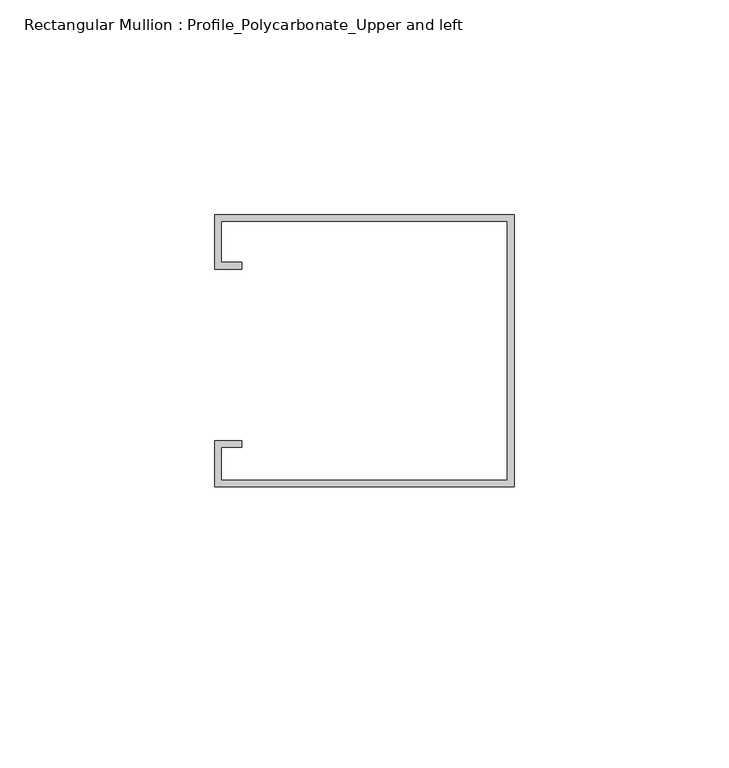
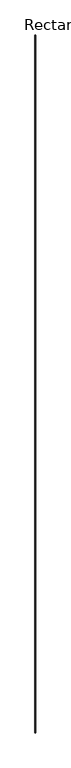
"""IFC4 building model written with IfcOpenShell, lengths in millimetres: member geometry, Rectangular Mullion : Profile_Polycarbonate_Upper and left."""

import ifcopenshell
import ifcopenshell.guid

model = None  # the IFC model being written
_history = None  # IfcOwnerHistory: only IFC2X3 demands one
_inside = {}  # id of a spatial element -> (the spatial element, [elements in it])
_under = {}  # id of a project, library or spatial element -> (it, [spatial elements below it])
_declared = {}  # id of a project -> (the project, [libraries it declares])
_typed = {}  # id of a type object -> (the type object, [elements of that type])
_made_of = {}  # id of a material, layer set ... -> (it, [elements and type objects made of it])


def new_model(schema):
    """Start an empty IFC model of exactly this schema.

    Asked for "IFC4X3", IfcOpenShell would pick the latest addendum, in which some entities
    have other attributes; the version numbers below select the first issue.
    IFC2X3 requires an IfcOwnerHistory on every rooted entity: one is made here for all.
    """
    global model, _history
    if schema == "IFC4X3":
        model = ifcopenshell.file(schema_version=(4, 3, 0, 0))
    else:
        model = ifcopenshell.file(schema=schema)
    _inside.clear()
    _under.clear()
    _declared.clear()
    _typed.clear()
    _made_of.clear()
    _history = None
    if model.schema == "IFC2X3":
        org = make("IfcOrganization", Name="unknown")
        user = make(
            "IfcPersonAndOrganization",
            ThePerson=make("IfcPerson", FamilyName="unknown"),
            TheOrganization=org,
        )
        app = make(
            "IfcApplication",
            ApplicationDeveloper=org,
            Version="unknown",
            ApplicationFullName="unknown",
            ApplicationIdentifier="unknown",
        )
        _history = make(
            "IfcOwnerHistory",
            OwningUser=user,
            OwningApplication=app,
            ChangeAction="ADDED",
            CreationDate=0,
        )
    return model


def make(cls, **values):
    """One entity of the class cls with the attributes given. An attribute that is None is left unset."""
    return model.create_entity(
        cls, **{name: value for name, value in values.items() if value is not None}
    )


def rooted(cls, **values):
    """An entity with a GlobalId (a new one), such as an element, a storey or a relation."""
    return make(cls, GlobalId=ifcopenshell.guid.new(), OwnerHistory=_history, **values)


def si_unit(unit_type, name, prefix=None):
    """IfcSIUnit, for example si_unit("LENGTHUNIT", "METRE", prefix="MILLI")."""
    return make("IfcSIUnit", UnitType=unit_type, Prefix=prefix, Name=name)


def assignment(units):
    """IfcUnitAssignment: the units of a project."""
    return None if units is None else make("IfcUnitAssignment", Units=units)


def point(xyz):
    """IfcCartesianPoint."""
    return None if xyz is None else make("IfcCartesianPoint", Coordinates=xyz)


def direction(xyz):
    """IfcDirection."""
    return None if xyz is None else make("IfcDirection", DirectionRatios=xyz)


def frame(location, z_axis=None, x_axis=None):
    """IfcAxis2Placement3D, a coordinate frame: its origin and axes. An axis left out is left unset."""
    return make(
        "IfcAxis2Placement3D",
        Location=point(location),
        Axis=direction(z_axis),
        RefDirection=direction(x_axis),
    )


def origin():
    """The frame at (0, 0, 0) with its axes left unset."""
    return frame((0.0, 0.0, 0.0))


def place(relative_to, where):
    """IfcLocalPlacement: puts the frame where relative to a parent placement (None: the world)."""
    return make(
        "IfcLocalPlacement", PlacementRelTo=relative_to, RelativePlacement=where
    )


def context(
    kind, dimensions, precision=None, world=None, true_north=None, identifier=None
):
    """IfcGeometricRepresentationContext, for example the 3D "Model" context."""
    return make(
        "IfcGeometricRepresentationContext",
        ContextIdentifier=identifier,
        ContextType=kind,
        CoordinateSpaceDimension=dimensions,
        Precision=precision,
        WorldCoordinateSystem=world,
        TrueNorth=true_north,
    )


def project(units=None, contexts=None):
    """IfcProject with its units and contexts."""
    return rooted(
        "IfcProject",
        Name="project",
        RepresentationContexts=contexts,
        UnitsInContext=assignment(units),
    )


def spatial(cls, under=None, at=None, **own):
    """A site, building, storey or space (cls), placed at a placement, below another one or the project."""
    s = rooted(cls, ObjectPlacement=at, **own)
    if under is not None:
        _under.setdefault(under.id(), (under, []))[1].append(s)
    return s


def polyline(points):
    """IfcPolyline through the points."""
    return make("IfcPolyline", Points=[point(p) for p in points])


def outline(outer, holes=None, kind="AREA"):
    """IfcArbitraryClosedProfileDef: a profile drawn as a closed curve; with holes, ...WithVoids."""
    if holes is None:
        return make("IfcArbitraryClosedProfileDef", ProfileType=kind, OuterCurve=outer)
    return make(
        "IfcArbitraryProfileDefWithVoids",
        ProfileType=kind,
        OuterCurve=outer,
        InnerCurves=holes,
    )


def extrude(swept, where, along, depth):
    """IfcExtrudedAreaSolid: the profile swept, set in the frame where, extruded along a direction by depth."""
    return make(
        "IfcExtrudedAreaSolid",
        SweptArea=swept,
        Position=where,
        ExtrudedDirection=direction(along),
        Depth=depth,
    )


def shape(context_of_items, identifier, shape_type, items):
    """IfcShapeRepresentation: the items that make up one representation, for example the "Body"."""
    return make(
        "IfcShapeRepresentation",
        ContextOfItems=context_of_items,
        RepresentationIdentifier=identifier,
        RepresentationType=shape_type,
        Items=items,
    )


def source(mapping_origin, context_of_items, identifier, shape_type, items):
    """IfcRepresentationMap: a shape defined once, which mapped items show again and again."""
    return make(
        "IfcRepresentationMap",
        MappingOrigin=mapping_origin,
        MappedRepresentation=shape(context_of_items, identifier, shape_type, items),
    )


def transform(
    local_origin,
    x_axis=None,
    y_axis=None,
    z_axis=None,
    scale=None,
    scale2=None,
    scale3=None,
    uniform=True,
):
    """IfcCartesianTransformationOperator3D, or its non-uniform kind. x_axis, y_axis, z_axis: its Axis1, 2, 3."""
    if uniform:
        return make(
            "IfcCartesianTransformationOperator3D",
            Axis1=direction(x_axis),
            Axis2=direction(y_axis),
            LocalOrigin=point(local_origin),
            Scale=scale,
            Axis3=direction(z_axis),
        )
    return make(
        "IfcCartesianTransformationOperator3DnonUniform",
        Axis1=direction(x_axis),
        Axis2=direction(y_axis),
        LocalOrigin=point(local_origin),
        Scale=scale,
        Axis3=direction(z_axis),
        Scale2=scale2,
        Scale3=scale3,
    )


def mapped(mapping_source, mapping_target):
    """IfcMappedItem: shows the shape of a source again, moved by a transform."""
    return make(
        "IfcMappedItem", MappingSource=mapping_source, MappingTarget=mapping_target
    )


def made_of(thing, what):
    """Note that an element or type object is made of a material, layer set ...; save() writes the relation."""
    if what is not None:
        _made_of.setdefault(what.id(), (what, []))[1].append(thing)
    return thing


def element(
    cls,
    number,
    at=None,
    inside=None,
    cuts=None,
    type_object=None,
    material=None,
    context=None,
    identifier="Body",
    shape_type=None,
    held_by="IfcProductDefinitionShape",
    body=None,
    shapes=None,
    **own,
):
    """One element of the class cls, such as IfcWall. Its Tag is "e" and its number.

    at: its placement. inside: the storey or other place that contains it. cuts: it is an
    opening in that element (IfcRelVoidsElement). A single representation is given by context,
    identifier, shape_type and body (its items); several are given by shapes. held_by: the class
    of the entity that holds the representations. save() writes the other relations.
    """
    e = rooted(cls, Tag="e%d" % number, ObjectPlacement=at, **own)
    if body is not None:
        shapes = [shape(context, identifier, shape_type, body)]
    if shapes is not None:
        e.Representation = make(held_by, Representations=shapes)
    if inside is not None:
        _inside.setdefault(inside.id(), (inside, []))[1].append(e)
    if cuts is not None:
        rooted(
            "IfcRelVoidsElement", RelatingBuildingElement=cuts, RelatedOpeningElement=e
        )
    if type_object is not None:
        _typed.setdefault(type_object.id(), (type_object, []))[1].append(e)
    return made_of(e, material)


def aggregate(whole, parts):
    """IfcRelAggregates: a whole, such as a stair, and the parts it consists of."""
    return rooted("IfcRelAggregates", RelatingObject=whole, RelatedObjects=parts)


def save(model, path):
    """Write the relations noted so far, then the file.

    IfcRelAggregates (storeys below a building ...), IfcRelContainedInSpatialStructure (elements
    in a storey), IfcRelDefinesByType, IfcRelAssociatesMaterial and IfcRelDeclares: one each for
    every whole, place, type object, material and project.
    """
    for whole, parts in _under.values():
        aggregate(whole, parts)
    for where, things in _inside.values():
        rooted(
            "IfcRelContainedInSpatialStructure",
            RelatedElements=things,
            RelatingStructure=where,
        )
    for kind, things in _typed.values():
        rooted("IfcRelDefinesByType", RelatedObjects=things, RelatingType=kind)
    for what, things in _made_of.values():
        rooted("IfcRelAssociatesMaterial", RelatedObjects=things, RelatingMaterial=what)
    for by, libraries in _declared.values():
        rooted("IfcRelDeclares", RelatingContext=by, RelatedDefinitions=libraries)
    model.write(path)


def rectangular_mullion_profile_polycarbonate_upper_and_left_92e5e834(model_context):
    return source(origin(), model_context, "Body", "SweptSolid", [
        extrude(outline(polyline([(0.0, 32.7), (0.0, -30.8), (-69.85, -30.8), (-69.85, -20.0), (-63.5, -20.0), (-63.5, -21.5875), (-68.2625, -21.5875), (-68.2625, -29.2125), (-1.5875, -29.2125), (-1.5875, 31.1125), (-68.2625, 31.1125), (-68.2625, 21.5875), (-63.5, 21.5875), (-63.5, 20.0), (-69.85, 20.0), (-69.85, 32.7), (0.0, 32.7)])), frame((0.0, 0.0, -88753.95), z_axis=(0.0, 0.0, 1.0), x_axis=(1.0, 0.0, 0.0)), (0.0, 0.0, 1.0), 88753.95),
    ])


if __name__ == "__main__":
    model = new_model("IFC4")
    model_context = context("Model", 3, world=origin())
    ifc_project = project(units=[si_unit("LENGTHUNIT", "METRE", prefix="MILLI")], contexts=[model_context])
    site = spatial("IfcSite", under=ifc_project)
    building = spatial("IfcBuilding", under=site)
    placement = place(None, origin())
    rectangular_mullion_profile_polycarbonate_upper_and_left_shape = rectangular_mullion_profile_polycarbonate_upper_and_left_92e5e834(model_context)
    element("IfcMember", 1, ObjectType="Rectangular Mullion : Profile_Polycarbonate_Upper and left", at=placement, inside=building, context=model_context, shape_type="MappedRepresentation", body=[
        mapped(rectangular_mullion_profile_polycarbonate_upper_and_left_shape, transform((0.0, 0.0, 0.0), x_axis=(1.0, 0.0, 0.0), y_axis=(0.0, 1.0, 0.0), z_axis=(0.0, 0.0, 1.0))),
    ])
    save(model, "model.ifc")

# Revit data of these elements
# Type "Rectangular Mullion : Profile_Polycarbonate_Upper and left"
#   built-in parameter 1007322 = 0.208333 (stored number, unit not read)
#   built-in parameter 1007321 = 0.00520833 (stored number, unit not read)
#   built-in parameter 1007320 = 0 (stored number, unit not read)
